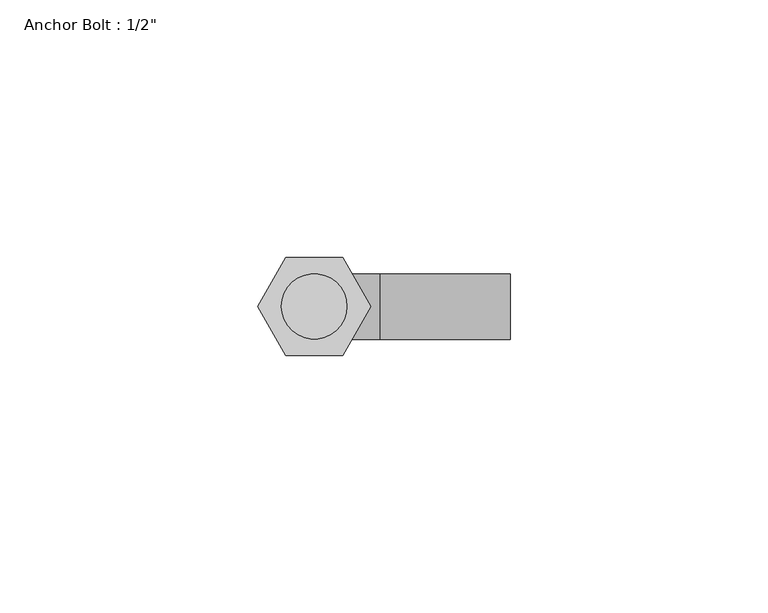
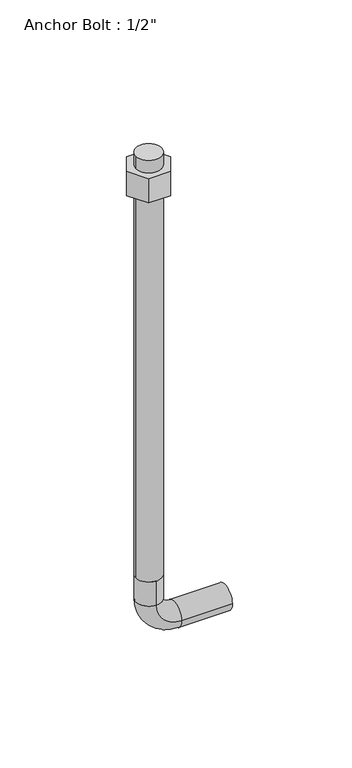
"""IFC4 building model written with IfcOpenShell, lengths in millimetres: fastener geometry."""

from ifc_helpers import new_model, si_unit, point, frame, origin, origin_with_axes, place, context, project, spatial, polyline, circle_curve, ellipse_curve, trimmed, outline, extrude, source, transform, mapped, element, save
from ifc_brep_helpers import plane_surface, cylinder_surface, revolved_surface, advanced_brep


def fastener_5f8ddbac(model_context):
    return source(origin(), model_context, "Body", "SolidModel", [
        advanced_brep(
        [(-6.35, 0.0, 19.05), (6.35, 0.0, 19.05), (-6.35, 0.0, -203.2), (0.0, -6.35, -203.2), (6.35, 0.0, -203.2), (0.0, 6.35, -203.2), (0.0, 6.35, -215.9), (0.0, -6.35, -215.9), (12.7, 6.35, -228.6), (12.7, -6.35, -228.6), (38.1, 6.35, -228.6), (38.1, -6.35, -228.6)],
        [
            (0, 1, circle_curve(frame((0.0, 0.0, 19.05), z_axis=(0.0, 0.0, 1.0), x_axis=(1.0, 0.0, 0.0)), 6.35)),
            (1, 0, circle_curve(frame((0.0, 0.0, 19.05), z_axis=(0.0, 0.0, 1.0), x_axis=(1.0, 0.0, 0.0)), 6.35)),
            (0, 2),
            (2, 3, circle_curve(frame((0.0, 0.0, -203.2), z_axis=(0.0, 0.0, 1.0), x_axis=(1.0, 0.0, 0.0)), 6.35)),
            (3, 4, circle_curve(frame((0.0, 0.0, -203.2), z_axis=(0.0, 0.0, 1.0), x_axis=(1.0, 0.0, 0.0)), 6.35)),
            (4, 1),
            (4, 5, circle_curve(frame((0.0, 0.0, -203.2), z_axis=(0.0, 0.0, 1.0), x_axis=(1.0, 0.0, 0.0)), 6.35)),
            (5, 2, circle_curve(frame((0.0, 0.0, -203.2), z_axis=(0.0, 0.0, 1.0), x_axis=(1.0, 0.0, 0.0)), 6.35)),
            (5, 6),
            (6, 7, circle_curve(frame((0.0, 0.0, -215.9), z_axis=(0.0, 0.0, 1.0), x_axis=(0.0, -1.0, 0.0)), 6.35)),
            (7, 3),
            (7, 6, circle_curve(frame((0.0, 0.0, -215.9), z_axis=(0.0, 0.0, 1.0), x_axis=(0.0, -1.0, 0.0)), 6.35)),
            (6, 8, circle_curve(frame((12.7, 6.35, -215.9), z_axis=(0.0, -1.0, 0.0), x_axis=(-1.0, 0.0, 0.0)), 12.7)),
            (8, 9, circle_curve(frame((12.7, 0.0, -228.6), z_axis=(-1.0, 0.0, 0.0), x_axis=(0.0, -1.0, 0.0)), 6.35)),
            (9, 7, circle_curve(frame((12.7, -6.35, -215.9), z_axis=(0.0, 1.0, 0.0), x_axis=(-1.0, 0.0, 0.0)), 12.7)),
            (9, 8, circle_curve(frame((12.7, 0.0, -228.6), z_axis=(-1.0, 0.0, 0.0), x_axis=(0.0, -1.0, 0.0)), 6.35)),
            (10, 11, circle_curve(frame((38.1, 0.0, -228.6), z_axis=(1.0, 0.0, 0.0), x_axis=(0.0, -1.0, 0.0)), 6.35)),
            (11, 10, circle_curve(frame((38.1, 0.0, -228.6), z_axis=(1.0, 0.0, 0.0), x_axis=(0.0, -1.0, 0.0)), 6.35)),
            (8, 10),
            (11, 9),
        ],
        [
            plane_surface(frame((6.35, 0.0, 19.05), z_axis=(0.0, 0.0, 1.0), x_axis=(0.0, 1.0, 0.0))),
            cylinder_surface(frame((0.0, 0.0, -203.2), z_axis=(0.0, 0.0, 1.0), x_axis=(1.0, 0.0, 0.0)), 6.35),
            cylinder_surface(frame((0.0, 0.0, -203.2), z_axis=(0.0, 0.0, 1.0), x_axis=(0.0, -1.0, 0.0)), 6.35),
            revolved_surface(trimmed(ellipse_curve(frame((0.0, 0.0, -215.9), z_axis=(0.0, 0.0, 1.0), x_axis=(0.0, -1.0, 0.0)), 6.35, 6.35), [point((0.0, 6.35, -215.9))], [point((0.0, -6.35, -215.9))], True, "CARTESIAN"), (12.7, 0.0, -215.9), (0.0, -1.0, 0.0)),
            revolved_surface(trimmed(ellipse_curve(frame((0.0, 0.0, -215.9), z_axis=(0.0, 0.0, 1.0), x_axis=(0.0, -1.0, 0.0)), 6.35, 6.35), [point((0.0, -6.35, -215.9))], [point((0.0, 6.35, -215.9))], True, "CARTESIAN"), (12.7, 0.0, -215.9), (0.0, -1.0, 0.0)),
            plane_surface(frame((38.1, 0.0, -228.6), z_axis=(1.0, 0.0, 0.0), x_axis=(0.0, -1.0, 0.0))),
            cylinder_surface(frame((12.7, 0.0, -228.6), z_axis=(-1.0, 0.0, 0.0), x_axis=(0.0, -1.0, 0.0)), 6.35),
        ],
        [
            (0, [[1, 2]]),
            (1, [[-1, 3, 4, 5, 6]]),
            (1, [[-2, -6, 7, 8, -3]]),
            (2, [[9, 10, 11, -4, -8]]),
            (2, [[-9, -7, -5, -11, 12]]),
            (3, [[-10, 13, 14, 15]]),
            (4, [[-12, -15, 16, -13]]),
            (5, [[17, 18]]),
            (6, [[-14, 19, -18, 20]]),
            (6, [[-16, -20, -17, -19]]),
        ],
    ),
        extrude(outline(polyline([(-10.9985226, 0.0), (-5.4992613, 9.525), (5.4992613, 9.525), (10.9985226, 0.0), (5.4992613, -9.525), (-5.4992613, -9.525), (-10.9985226, 0.0)])), origin_with_axes(), (0.0, 0.0, 1.0), 12.7),
    ])


if __name__ == "__main__":
    model = new_model("IFC4")
    model_context = context("Model", 3, world=origin())
    ifc_project = project(units=[si_unit("LENGTHUNIT", "METRE", prefix="MILLI")], contexts=[model_context])
    site = spatial("IfcSite", under=ifc_project)
    building = spatial("IfcBuilding", under=site)
    placement = place(None, origin())
    fastener_shape = fastener_5f8ddbac(model_context)
    element("IfcFastener", 1, ObjectType="Anchor Bolt : 1/2\"", at=placement, inside=building, context=model_context, shape_type="MappedRepresentation", body=[
        mapped(fastener_shape, transform((0.0, 0.0, 0.0), x_axis=(1.0, 0.0, 0.0), y_axis=(0.0, 1.0, 0.0), z_axis=(0.0, 0.0, 1.0))),
    ])
    save(model, "model.ifc")

# Revit data of these elements
# Type "Anchor Bolt : 1/2\""
#   Side = 0' - 0 111/256"
#   Radius = 0' - 0 1/4"
#   Length = 0' - 8"
#   Head Size = 0' - 0 3/4"
#   Head Radius = 0' - 0 3/8"
#   Head Height = 0' - 0 1/2"
#   Diameter = 0' - 0 1/2"
#   Default Elevation = 4' - 0"
#   Bolt Material (Size) = 1/2" ANCHOR BOLTS (7" MIN. EMBED) AT 72" MIN O.C. SPACING (18" MAX. FROM CORNERS)
# Element 1 (IfcFastener, "Anchor Bolt : 1/2\"")
#   Materials on its faces: "1/2\" ANCHOR BOLTS (7\" MIN. EMBED) AT 72\" MIN O.C. SPACING (18\" MAX. FROM CORNERS)"
# Materials
#   "1/2\" ANCHOR BOLTS (7\" MIN. EMBED) AT 72\" MIN O.C. SPACING (18\" MAX. FROM CORNERS)": class "Generic", colour RGB 120 120 120, transparency 0, Cost = 0
